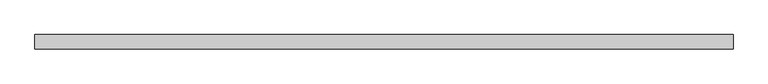
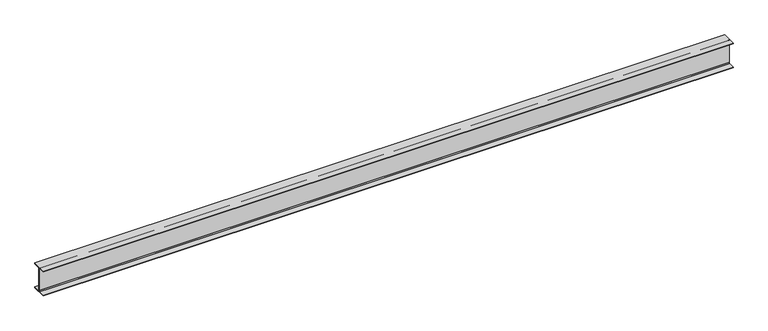
"""IFC4 building model written with IfcOpenShell, lengths in millimetres: beam geometry, Old_Steel Beam_H-KSD3502 : H_SB_ASB_H-390×300x10x16."""

from ifc_helpers import new_model, si_unit, point, frame, frame_2d, origin, place, context, project, spatial, polyline, circle_curve, trimmed, segment, composite_curve, outline, extrude, source, transform, mapped, element, save


def beam_be96817d(model_context):
    return source(origin(), model_context, "Body", "SweptSolid", [
        extrude(outline(composite_curve([segment(polyline([(82.5, -141.5), (82.5, -151.7), (-82.5, -151.7), (-82.5, -141.5), (-11.9, -141.5)]), True, "CONTINUOUS"), segment(trimmed(circle_curve(frame_2d((-11.9, -132.6)), 8.9), [point((-11.9, -141.5))], [point((-3.0, -132.6))], True, "CARTESIAN"), True, "CONTINUOUS"), segment(polyline([(-3.0, -132.6), (-3.0, 132.6)]), True, "CONTINUOUS"), segment(trimmed(circle_curve(frame_2d((-11.9, 132.6)), 8.9), [point((-3.0, 132.6))], [point((-11.9, 141.5))], True, "CARTESIAN"), True, "CONTINUOUS"), segment(polyline([(-11.9, 141.5), (-82.5, 141.5), (-82.5, 151.7), (82.5, 151.7), (82.5, 141.5), (11.9, 141.5)]), True, "CONTINUOUS"), segment(trimmed(circle_curve(frame_2d((11.9, 132.6)), 8.9), [point((11.9, 141.5))], [point((3.0, 132.6))], True, "CARTESIAN"), True, "CONTINUOUS"), segment(polyline([(3.0, 132.6), (3.0, -132.6)]), True, "CONTINUOUS"), segment(trimmed(circle_curve(frame_2d((11.9, -132.6)), 8.9), [point((3.0, -132.6))], [point((11.9, -141.5))], True, "CARTESIAN"), True, "CONTINUOUS"), segment(polyline([(11.9, -141.5), (82.5, -141.5)]), True, "CONTINUOUS")], self_intersect=False)), frame((-3987.2999994, 0.0, 0.0), z_axis=(1.0, 0.0, 0.0), x_axis=(0.0, 1.0, 0.0)), (0.0, 0.0, 1.0), 7974.5999988),
    ])


if __name__ == "__main__":
    model = new_model("IFC4")
    model_context = context("Model", 3, world=origin())
    ifc_project = project(units=[si_unit("LENGTHUNIT", "METRE", prefix="MILLI")], contexts=[model_context])
    site = spatial("IfcSite", under=ifc_project)
    building = spatial("IfcBuilding", under=site)
    placement = place(None, origin())
    beam_shape = beam_be96817d(model_context)
    element("IfcBeam", 1, ObjectType="Old_Steel Beam_H-KSD3502 : H_SB_ASB_H-390×300x10x16", at=placement, inside=building, context=model_context, shape_type="MappedRepresentation", body=[
        mapped(beam_shape, transform((0.0, 0.0, 0.0), x_axis=(1.0, 0.0, 0.0), y_axis=(0.0, 1.0, 0.0), z_axis=(0.0, 0.0, 1.0))),
    ])
    save(model, "model.ifc")

# Revit data of these elements
# Type "Old_Steel Beam_H-KSD3502 : H_SB_ASB_H-390×300x10x16"
#   Width = 30.0 cm
#   Web Thickness = 1.0 cm
#   Web Fillet = 2.2 cm
#   Warping Constant = 2517770.0 cm⁶
#   Torsional Moment of Inertia = 94.3867 cm⁴
#   Torsional Modulus = 1.0 cm³
#   Section Area = 136.0 cm²
#   Plastic Modulus weak axis = 733.0 cm³
#   Plastic Modulus strong axis = 2190.0 cm³
#   Perimeter = 1.92 m²/m
#   Nominal Weight = 107.00 kgf/m
#   Moment of Inertia weak axis = 7210.00 cm⁴
#   Moment of Inertia strong axis = 38700.00 cm⁴
#   Height = 39.0 cm
#   Flange Thickness = 1.6 cm
#   Elastic Modulus weak axis = 481.0 cm³
#   Elastic Modulus strong axis = 1980.0 cm³
#   Centroid Vertical = 19.5 cm
#   Centroid Horizontal = 15.0 cm
#   Length [instance default] = 1.5240 m
#   Structural Material [instance default] = Steel, 45-345
#   Assembly Code = ""
# Element 1 (IfcBeam, "Old_Steel Beam_H-KSD3502 : H_SB_ASB_H-390×300x10x16")
#   Structural Material = none
# Materials
#   "Steel, 45-345": class "Metal", colour RGB 189 187 185, transparency 0, Description = "Steel 345 MPa", Cost = 0
